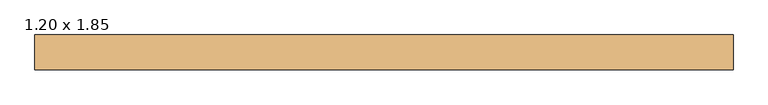
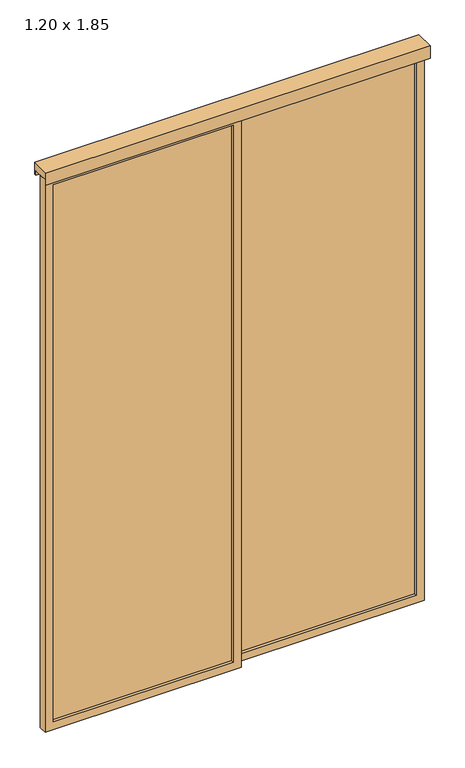
"""IFC4 building model written with IfcOpenShell, lengths in millimetres: door geometry, CC_ND-200_BOX-BANHEIRO : 1.20 x 1.85."""

import ifcopenshell
import ifcopenshell.guid

model = None  # the IFC model being written
_history = None  # IfcOwnerHistory: only IFC2X3 demands one
_inside = {}  # id of a spatial element -> (the spatial element, [elements in it])
_under = {}  # id of a project, library or spatial element -> (it, [spatial elements below it])
_declared = {}  # id of a project -> (the project, [libraries it declares])
_typed = {}  # id of a type object -> (the type object, [elements of that type])
_made_of = {}  # id of a material, layer set ... -> (it, [elements and type objects made of it])


def new_model(schema):
    """Start an empty IFC model of exactly this schema.

    Asked for "IFC4X3", IfcOpenShell would pick the latest addendum, in which some entities
    have other attributes; the version numbers below select the first issue.
    IFC2X3 requires an IfcOwnerHistory on every rooted entity: one is made here for all.
    """
    global model, _history
    if schema == "IFC4X3":
        model = ifcopenshell.file(schema_version=(4, 3, 0, 0))
    else:
        model = ifcopenshell.file(schema=schema)
    _inside.clear()
    _under.clear()
    _declared.clear()
    _typed.clear()
    _made_of.clear()
    _history = None
    if model.schema == "IFC2X3":
        org = make("IfcOrganization", Name="unknown")
        user = make(
            "IfcPersonAndOrganization",
            ThePerson=make("IfcPerson", FamilyName="unknown"),
            TheOrganization=org,
        )
        app = make(
            "IfcApplication",
            ApplicationDeveloper=org,
            Version="unknown",
            ApplicationFullName="unknown",
            ApplicationIdentifier="unknown",
        )
        _history = make(
            "IfcOwnerHistory",
            OwningUser=user,
            OwningApplication=app,
            ChangeAction="ADDED",
            CreationDate=0,
        )
    return model


def make(cls, **values):
    """One entity of the class cls with the attributes given. An attribute that is None is left unset."""
    return model.create_entity(
        cls, **{name: value for name, value in values.items() if value is not None}
    )


def rooted(cls, **values):
    """An entity with a GlobalId (a new one), such as an element, a storey or a relation."""
    return make(cls, GlobalId=ifcopenshell.guid.new(), OwnerHistory=_history, **values)


def si_unit(unit_type, name, prefix=None):
    """IfcSIUnit, for example si_unit("LENGTHUNIT", "METRE", prefix="MILLI")."""
    return make("IfcSIUnit", UnitType=unit_type, Prefix=prefix, Name=name)


def assignment(units):
    """IfcUnitAssignment: the units of a project."""
    return None if units is None else make("IfcUnitAssignment", Units=units)


def point(xyz):
    """IfcCartesianPoint."""
    return None if xyz is None else make("IfcCartesianPoint", Coordinates=xyz)


def direction(xyz):
    """IfcDirection."""
    return None if xyz is None else make("IfcDirection", DirectionRatios=xyz)


def frame(location, z_axis=None, x_axis=None):
    """IfcAxis2Placement3D, a coordinate frame: its origin and axes. An axis left out is left unset."""
    return make(
        "IfcAxis2Placement3D",
        Location=point(location),
        Axis=direction(z_axis),
        RefDirection=direction(x_axis),
    )


def origin():
    """The frame at (0, 0, 0) with its axes left unset."""
    return frame((0.0, 0.0, 0.0))


def place(relative_to, where):
    """IfcLocalPlacement: puts the frame where relative to a parent placement (None: the world)."""
    return make(
        "IfcLocalPlacement", PlacementRelTo=relative_to, RelativePlacement=where
    )


def context(
    kind, dimensions, precision=None, world=None, true_north=None, identifier=None
):
    """IfcGeometricRepresentationContext, for example the 3D "Model" context."""
    return make(
        "IfcGeometricRepresentationContext",
        ContextIdentifier=identifier,
        ContextType=kind,
        CoordinateSpaceDimension=dimensions,
        Precision=precision,
        WorldCoordinateSystem=world,
        TrueNorth=true_north,
    )


def project(units=None, contexts=None):
    """IfcProject with its units and contexts."""
    return rooted(
        "IfcProject",
        Name="project",
        RepresentationContexts=contexts,
        UnitsInContext=assignment(units),
    )


def spatial(cls, under=None, at=None, **own):
    """A site, building, storey or space (cls), placed at a placement, below another one or the project."""
    s = rooted(cls, ObjectPlacement=at, **own)
    if under is not None:
        _under.setdefault(under.id(), (under, []))[1].append(s)
    return s


def polyline(points):
    """IfcPolyline through the points."""
    return make("IfcPolyline", Points=[point(p) for p in points])


def outline(outer, holes=None, kind="AREA"):
    """IfcArbitraryClosedProfileDef: a profile drawn as a closed curve; with holes, ...WithVoids."""
    if holes is None:
        return make("IfcArbitraryClosedProfileDef", ProfileType=kind, OuterCurve=outer)
    return make(
        "IfcArbitraryProfileDefWithVoids",
        ProfileType=kind,
        OuterCurve=outer,
        InnerCurves=holes,
    )


def extrude(swept, where, along, depth):
    """IfcExtrudedAreaSolid: the profile swept, set in the frame where, extruded along a direction by depth."""
    return make(
        "IfcExtrudedAreaSolid",
        SweptArea=swept,
        Position=where,
        ExtrudedDirection=direction(along),
        Depth=depth,
    )


def faces_of(points, faces, orient=None, outer=None):
    """IfcFace entities. A face is a list of loops; a loop is a list of indices into points, from 0.

    orient and outer hold one flag for each loop. By default every Orientation is true, the
    first loop of a face is its IfcFaceOuterBound and the others are IfcFaceBound.
    """
    made = []
    for i, loops in enumerate(faces):
        bounds = []
        for j, loop in enumerate(loops):
            is_outer = j == 0 if outer is None else outer[i][j]
            bounds.append(
                make(
                    "IfcFaceOuterBound" if is_outer else "IfcFaceBound",
                    Bound=make("IfcPolyLoop", Polygon=[points[k] for k in loop]),
                    Orientation=True if orient is None else orient[i][j],
                )
            )
        made.append(make("IfcFace", Bounds=bounds))
    return made


def faceted_brep(points, faces, orient=None, outer=None, voids=None):
    """IfcFacetedBrep: a solid bounded by flat faces; with voids (closed shells), ...WithVoids."""
    shared = [point(p) for p in points]
    hull = make("IfcClosedShell", CfsFaces=faces_of(shared, faces, orient, outer))
    if voids is None:
        return make("IfcFacetedBrep", Outer=hull)
    return make(
        "IfcFacetedBrepWithVoids",
        Outer=hull,
        Voids=[
            make(cls, CfsFaces=faces_of(shared, fs, o, b)) for cls, fs, o, b in voids
        ],
    )


def shape(context_of_items, identifier, shape_type, items):
    """IfcShapeRepresentation: the items that make up one representation, for example the "Body"."""
    return make(
        "IfcShapeRepresentation",
        ContextOfItems=context_of_items,
        RepresentationIdentifier=identifier,
        RepresentationType=shape_type,
        Items=items,
    )


def source(mapping_origin, context_of_items, identifier, shape_type, items):
    """IfcRepresentationMap: a shape defined once, which mapped items show again and again."""
    return make(
        "IfcRepresentationMap",
        MappingOrigin=mapping_origin,
        MappedRepresentation=shape(context_of_items, identifier, shape_type, items),
    )


def transform(
    local_origin,
    x_axis=None,
    y_axis=None,
    z_axis=None,
    scale=None,
    scale2=None,
    scale3=None,
    uniform=True,
):
    """IfcCartesianTransformationOperator3D, or its non-uniform kind. x_axis, y_axis, z_axis: its Axis1, 2, 3."""
    if uniform:
        return make(
            "IfcCartesianTransformationOperator3D",
            Axis1=direction(x_axis),
            Axis2=direction(y_axis),
            LocalOrigin=point(local_origin),
            Scale=scale,
            Axis3=direction(z_axis),
        )
    return make(
        "IfcCartesianTransformationOperator3DnonUniform",
        Axis1=direction(x_axis),
        Axis2=direction(y_axis),
        LocalOrigin=point(local_origin),
        Scale=scale,
        Axis3=direction(z_axis),
        Scale2=scale2,
        Scale3=scale3,
    )


def mapped(mapping_source, mapping_target):
    """IfcMappedItem: shows the shape of a source again, moved by a transform."""
    return make(
        "IfcMappedItem", MappingSource=mapping_source, MappingTarget=mapping_target
    )


def made_of(thing, what):
    """Note that an element or type object is made of a material, layer set ...; save() writes the relation."""
    if what is not None:
        _made_of.setdefault(what.id(), (what, []))[1].append(thing)
    return thing


def element(
    cls,
    number,
    at=None,
    inside=None,
    cuts=None,
    type_object=None,
    material=None,
    context=None,
    identifier="Body",
    shape_type=None,
    held_by="IfcProductDefinitionShape",
    body=None,
    shapes=None,
    **own,
):
    """One element of the class cls, such as IfcWall. Its Tag is "e" and its number.

    at: its placement. inside: the storey or other place that contains it. cuts: it is an
    opening in that element (IfcRelVoidsElement). A single representation is given by context,
    identifier, shape_type and body (its items); several are given by shapes. held_by: the class
    of the entity that holds the representations. save() writes the other relations.
    """
    e = rooted(cls, Tag="e%d" % number, ObjectPlacement=at, **own)
    if body is not None:
        shapes = [shape(context, identifier, shape_type, body)]
    if shapes is not None:
        e.Representation = make(held_by, Representations=shapes)
    if inside is not None:
        _inside.setdefault(inside.id(), (inside, []))[1].append(e)
    if cuts is not None:
        rooted(
            "IfcRelVoidsElement", RelatingBuildingElement=cuts, RelatedOpeningElement=e
        )
    if type_object is not None:
        _typed.setdefault(type_object.id(), (type_object, []))[1].append(e)
    return made_of(e, material)


def aggregate(whole, parts):
    """IfcRelAggregates: a whole, such as a stair, and the parts it consists of."""
    return rooted("IfcRelAggregates", RelatingObject=whole, RelatedObjects=parts)


def save(model, path):
    """Write the relations noted so far, then the file.

    IfcRelAggregates (storeys below a building ...), IfcRelContainedInSpatialStructure (elements
    in a storey), IfcRelDefinesByType, IfcRelAssociatesMaterial and IfcRelDeclares: one each for
    every whole, place, type object, material and project.
    """
    for whole, parts in _under.values():
        aggregate(whole, parts)
    for where, things in _inside.values():
        rooted(
            "IfcRelContainedInSpatialStructure",
            RelatedElements=things,
            RelatingStructure=where,
        )
    for kind, things in _typed.values():
        rooted("IfcRelDefinesByType", RelatedObjects=things, RelatingType=kind)
    for what, things in _made_of.values():
        rooted("IfcRelAssociatesMaterial", RelatedObjects=things, RelatingMaterial=what)
    for by, libraries in _declared.values():
        rooted("IfcRelDeclares", RelatingContext=by, RelatedDefinitions=libraries)
    model.write(path)


def door_1_20_x_1_85_7a0dc905(model_context):
    return source(origin(), model_context, "Body", "SolidModel", [
        extrude(outline(polyline([(602.5, 15.0), (602.5, 10.0), (10.0, 10.0), (10.0, 15.0), (602.5, 15.0)])), frame((0.0, 0.0, 10.0), z_axis=(0.0, 0.0, 1.0), x_axis=(1.0, 0.0, 0.0)), (0.0, 0.0, 1.0), 1805.0),
        faceted_brep([(587.5, 15.0, 1800.0), (587.5, 25.0, 1800.0), (587.5, 25.0, 25.0), (587.5, 15.0, 25.0), (612.5, 25.0, 1825.0), (612.5, 25.0, 0.0), (0.0, 25.0, 0.0), (0.0, 25.0, 1825.0), (25.0, 25.0, 1800.0), (25.0, 25.0, 25.0), (25.0, 15.0, 25.0), (10.0, 15.0, 1815.0), (10.0, 15.0, 10.0), (602.5, 15.0, 10.0), (602.5, 15.0, 1815.0), (25.0, 15.0, 1800.0), (612.5, 0.0, 1825.0), (612.5, 0.0, 0.0), (0.0, 0.0, 1825.0), (0.0, 0.0, 0.0), (587.5, 0.0, 1800.0), (587.5, 0.0, 25.0), (25.0, 0.0, 25.0), (25.0, 0.0, 1800.0), (587.5, 10.0, 1800.0), (587.5, 10.0, 25.0), (25.0, 10.0, 25.0), (25.0, 10.0, 1800.0), (602.5, 10.0, 1815.0), (602.5, 10.0, 10.0), (10.0, 10.0, 10.0), (10.0, 10.0, 1815.0)], [[[0, 1, 2, 3]], [[4, 5, 6, 7], [8, 9, 2, 1]], [[3, 2, 9, 10]], [[11, 12, 13, 14], [0, 3, 10, 15]], [[4, 16, 17, 5]], [[18, 19, 17, 16], [20, 21, 22, 23]], [[5, 17, 19, 6]], [[10, 9, 8, 15]], [[6, 19, 18, 7]], [[20, 24, 25, 21]], [[21, 25, 26, 22]], [[22, 26, 27, 23]], [[28, 14, 13, 29]], [[29, 13, 12, 30]], [[28, 29, 30, 31], [27, 26, 25, 24]], [[30, 12, 11, 31]], [[15, 8, 1, 0]], [[7, 18, 16, 4]], [[31, 11, 14, 28]], [[23, 27, 24, 20]]]),
        extrude(outline(polyline([(1190.0, 40.0), (1190.0, 35.0), (597.5, 35.0), (597.5, 40.0), (1190.0, 40.0)])), frame((0.0, 0.0, 10.0), z_axis=(0.0, 0.0, 1.0), x_axis=(1.0, 0.0, 0.0)), (0.0, 0.0, 1.0), 1805.0),
        faceted_brep([(1175.0, 40.0, 1800.0), (1175.0, 50.0, 1800.0), (1175.0, 50.0, 25.0), (1175.0, 40.0, 25.0), (1200.0, 50.0, 1825.0), (1200.0, 50.0, 0.0), (587.5, 50.0, 0.0), (587.5, 50.0, 1825.0), (612.5, 50.0, 1800.0), (612.5, 50.0, 25.0), (612.5, 40.0, 25.0), (597.5, 40.0, 1815.0), (597.5, 40.0, 10.0), (1190.0, 40.0, 10.0), (1190.0, 40.0, 1815.0), (612.5, 40.0, 1800.0), (1200.0, 25.0, 1825.0), (1200.0, 25.0, 0.0), (587.5, 25.0, 1825.0), (587.5, 25.0, 0.0), (1175.0, 25.0, 1800.0), (1175.0, 25.0, 25.0), (612.5, 25.0, 25.0), (612.5, 25.0, 1800.0), (1175.0, 35.0, 1800.0), (1175.0, 35.0, 25.0), (612.5, 35.0, 25.0), (612.5, 35.0, 1800.0), (1190.0, 35.0, 1815.0), (1190.0, 35.0, 10.0), (597.5, 35.0, 10.0), (597.5, 35.0, 1815.0)], [[[0, 1, 2, 3]], [[4, 5, 6, 7], [8, 9, 2, 1]], [[3, 2, 9, 10]], [[11, 12, 13, 14], [0, 3, 10, 15]], [[4, 16, 17, 5]], [[18, 19, 17, 16], [20, 21, 22, 23]], [[5, 17, 19, 6]], [[10, 9, 8, 15]], [[6, 19, 18, 7]], [[20, 24, 25, 21]], [[21, 25, 26, 22]], [[22, 26, 27, 23]], [[28, 14, 13, 29]], [[29, 13, 12, 30]], [[28, 29, 30, 31], [27, 26, 25, 24]], [[30, 12, 11, 31]], [[15, 8, 1, 0]], [[7, 18, 16, 4]], [[31, 11, 14, 28]], [[23, 27, 24, 20]]]),
        extrude(outline(polyline([(-5.0, 1810.0), (-5.0, 1850.0), (55.0, 1850.0), (55.0, 1810.0), (50.0, 1810.0), (50.0, 1825.0), (0.0, 1825.0), (0.0, 1810.0), (-5.0, 1810.0)])), frame((0.0, 0.0, 0.0), z_axis=(1.0, 0.0, 0.0), x_axis=(0.0, 1.0, 0.0)), (0.0, 0.0, 1.0), 1200.0),
    ])


if __name__ == "__main__":
    model = new_model("IFC4")
    model_context = context("Model", 3, world=origin())
    ifc_project = project(units=[si_unit("LENGTHUNIT", "METRE", prefix="MILLI")], contexts=[model_context])
    site = spatial("IfcSite", under=ifc_project)
    building = spatial("IfcBuilding", under=site)
    placement = place(None, origin())
    door_1_20_x_1_85_shape = door_1_20_x_1_85_7a0dc905(model_context)
    element("IfcDoor", 1, ObjectType="CC_ND-200_BOX-BANHEIRO : 1.20 x 1.85", at=placement, inside=building, context=model_context, shape_type="MappedRepresentation", body=[
        mapped(door_1_20_x_1_85_shape, transform((0.0, 0.0, 0.0), x_axis=(1.0, 0.0, 0.0), y_axis=(0.0, 1.0, 0.0), z_axis=(0.0, 0.0, 1.0))),
    ])
    save(model, "model.ifc")

# Revit data of these elements
# Type "CC_ND-200_BOX-BANHEIRO : 1.20 x 1.85"
#   Type Mark = "145"
#   Width = 1.20 m
#   Material montante = Aluminio
#   Materia vidro = Vidro
# Element 1 (IfcDoor, "CC_ND-200_BOX-BANHEIRO : 1.20 x 1.85")
#   Materials on its faces: "Aluminio", "Vidro"
# Materials
#   "Aluminio": class "Genérico", colour RGB 120 120 120, transparency 0, Cost = 0
#   "Vidro": class "Vidro", colour RGB 230 230 230, transparency 0.75, Description = "JANELA COM 04 FOLHAS DE CORRER E VIDRO TRANSPARENTE 6mm", Cost = 0
